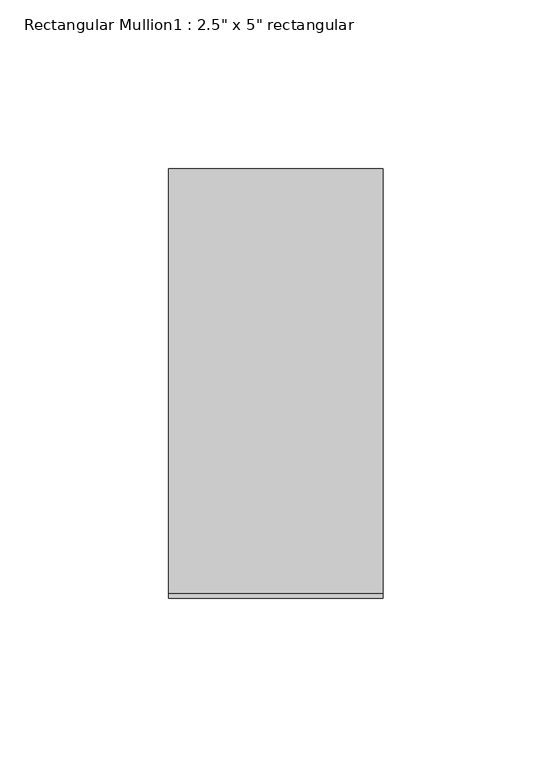
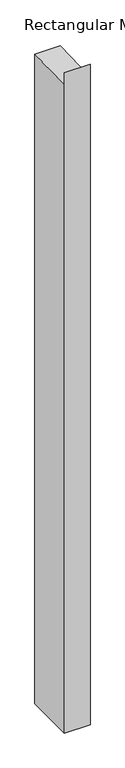
"""IFC4 building model written with IfcOpenShell, lengths in millimetres: member geometry."""

from ifc_helpers import new_model, si_unit, frame, origin, place, context, project, spatial, polyline, outline, extrude, source, transform, mapped, element, save


def member_78ef575d(model_context):
    return source(origin(), model_context, "Body", "SweptSolid", [
        extrude(outline(polyline([(-63.5, 30.4964474), (-62.1974623, -2.4813918), (63.5, 2.4833266), (63.5, -1702.5398307), (-63.5, -1702.5398307), (-63.5, 30.4964474)])), frame((-63.5, 0.0, 0.0), z_axis=(1.0, 0.0, 0.0), x_axis=(0.0, 1.0, 0.0)), (0.0, 0.0, 1.0), 63.5),
    ])


if __name__ == "__main__":
    model = new_model("IFC4")
    model_context = context("Model", 3, world=origin())
    ifc_project = project(units=[si_unit("LENGTHUNIT", "METRE", prefix="MILLI")], contexts=[model_context])
    site = spatial("IfcSite", under=ifc_project)
    building = spatial("IfcBuilding", under=site)
    placement = place(None, origin())
    member_shape = member_78ef575d(model_context)
    element("IfcMember", 1, ObjectType="Rectangular Mullion1 : 2.5\" x 5\" rectangular", at=placement, inside=building, context=model_context, shape_type="MappedRepresentation", body=[
        mapped(member_shape, transform((0.0, 0.0, 0.0), x_axis=(1.0, 0.0, 0.0), y_axis=(0.0, 1.0, 0.0), z_axis=(0.0, 0.0, 1.0))),
    ])
    save(model, "model.ifc")

# Revit data of these elements
# Type "Rectangular Mullion1 : 2.5\" x 5\" rectangular"
#   built-in parameter 1007304 = 0.416667 (stored number, unit not read)
#   built-in parameter 1007301 = 0.104167 (stored number, unit not read)
#   built-in parameter 1007300 = 0.104167 (stored number, unit not read)
# Element 1 (IfcMember, "Rectangular Mullion1 : 2.5\" x 5\" rectangular")
#   Materials on its faces: "support-frame"
# Materials
#   "support-frame": class "Unassigned", colour RGB 233 233 233, transparency 0, Cost = 0
